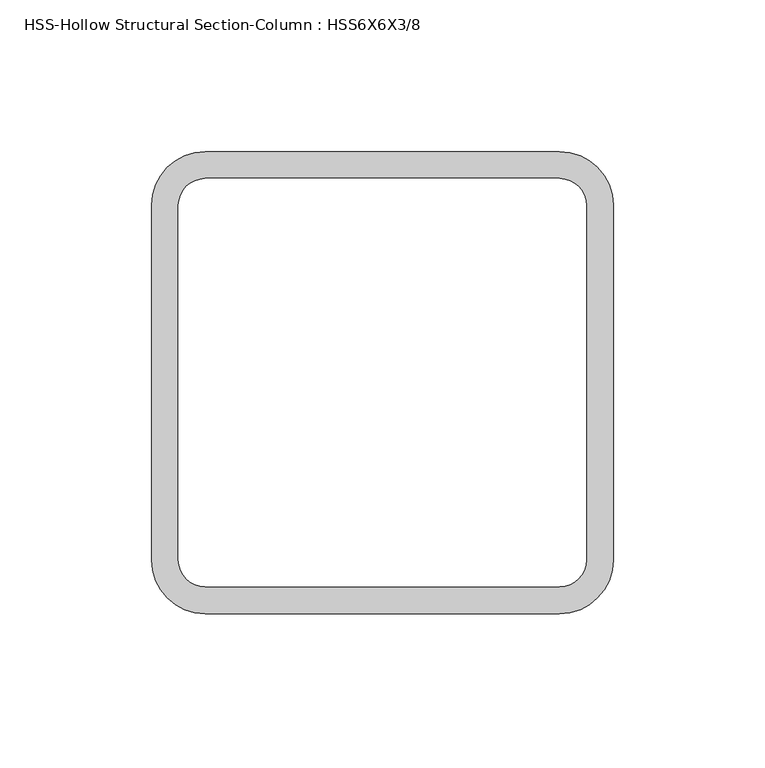
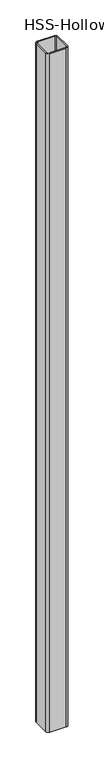
"""IFC4 building model written with IfcOpenShell, lengths in millimetres: column geometry, HSS-Hollow Structural Section-Column : HSS6X6X3/8."""

from ifc_helpers import new_model, si_unit, point, frame, frame_2d, origin, place, context, project, spatial, polyline, circle_curve, trimmed, segment, composite_curve, outline, extrude, source, transform, mapped, element, save


def hss_hollow_structural_section_column_hss6x6x3_8_7760a8ad(model_context):
    return source(origin(), model_context, "Body", "SweptSolid", [
        extrude(outline(composite_curve([segment(trimmed(circle_curve(frame_2d((58.4708, 58.4708)), 17.7292), [point((58.4708, 76.2))], [point((76.2, 58.4708))], False, "CARTESIAN"), True, "CONTINUOUS"), segment(polyline([(76.2, 58.4708), (76.2, -58.4708)]), True, "CONTINUOUS"), segment(trimmed(circle_curve(frame_2d((58.4708, -58.4708)), 17.7292), [point((76.2, -58.4708))], [point((58.4708, -76.2))], False, "CARTESIAN"), True, "CONTINUOUS"), segment(polyline([(58.4708, -76.2), (-58.4708, -76.2)]), True, "CONTINUOUS"), segment(trimmed(circle_curve(frame_2d((-58.4708, -58.4708)), 17.7292), [point((-58.4708, -76.2))], [point((-76.2, -58.4708))], False, "CARTESIAN"), True, "CONTINUOUS"), segment(polyline([(-76.2, -58.4708), (-76.2, 58.4708)]), True, "CONTINUOUS"), segment(trimmed(circle_curve(frame_2d((-58.4708, 58.4708)), 17.7292), [point((-76.2, 58.4708))], [point((-58.4708, 76.2))], False, "CARTESIAN"), True, "CONTINUOUS"), segment(polyline([(-58.4708, 76.2), (58.4708, 76.2)]), True, "CONTINUOUS")], self_intersect=False), holes=[composite_curve([segment(polyline([(58.4708, 67.3354), (-58.4708, 67.3354)]), True, "CONTINUOUS"), segment(trimmed(circle_curve(frame_2d((-58.4708, 58.4708)), 8.8646), [point((-58.4708, 67.3354))], [point((-67.3354, 58.4708))], True, "CARTESIAN"), True, "CONTINUOUS"), segment(polyline([(-67.3354, 58.4708), (-67.3354, -58.4708)]), True, "CONTINUOUS"), segment(trimmed(circle_curve(frame_2d((-58.4708, -58.4708)), 8.8646), [point((-67.3354, -58.4708))], [point((-58.4708, -67.3354))], True, "CARTESIAN"), True, "CONTINUOUS"), segment(polyline([(-58.4708, -67.3354), (58.4708, -67.3354)]), True, "CONTINUOUS"), segment(trimmed(circle_curve(frame_2d((58.4708, -58.4708)), 8.8646), [point((58.4708, -67.3354))], [point((67.3354, -58.4708))], True, "CARTESIAN"), True, "CONTINUOUS"), segment(polyline([(67.3354, -58.4708), (67.3354, 58.4708)]), True, "CONTINUOUS"), segment(trimmed(circle_curve(frame_2d((58.4708, 58.4708)), 8.8646), [point((67.3354, 58.4708))], [point((58.4708, 67.3354))], True, "CARTESIAN"), True, "CONTINUOUS")], self_intersect=False)]), frame((0.0, 0.0, 12566.65), z_axis=(0.0, 0.0, 1.0), x_axis=(1.0, 0.0, 0.0)), (0.0, 0.0, 1.0), 5060.95),
    ])


if __name__ == "__main__":
    model = new_model("IFC4")
    model_context = context("Model", 3, world=origin())
    ifc_project = project(units=[si_unit("LENGTHUNIT", "METRE", prefix="MILLI")], contexts=[model_context])
    site = spatial("IfcSite", under=ifc_project)
    building = spatial("IfcBuilding", under=site)
    placement = place(None, origin())
    hss_hollow_structural_section_column_hss6x6x3_8_shape = hss_hollow_structural_section_column_hss6x6x3_8_7760a8ad(model_context)
    element("IfcColumn", 1, ObjectType="HSS-Hollow Structural Section-Column : HSS6X6X3/8", at=placement, inside=building, context=model_context, shape_type="MappedRepresentation", body=[
        mapped(hss_hollow_structural_section_column_hss6x6x3_8_shape, transform((0.0, 0.0, 0.0), x_axis=(1.0, 0.0, 0.0), y_axis=(0.0, 1.0, 0.0), z_axis=(0.0, 0.0, 1.0))),
    ])
    save(model, "model.ifc")

# Revit data of these elements
# Type "HSS-Hollow Structural Section-Column : HSS6X6X3/8"
#   Assembly Code = "B10"
#   Shape = "Square"
#   W = 27.4
#   Ht = 0' - 6"
#   b = 0' - 6"
#   kr = 0' - 0.698"
#   t = 0' - 0.349"
#   A = 0.0526389 SF
#   Structural Material [instance default] = Steel ASTM A500, Grade B, Rectangular and Square
# Element 1 (IfcColumn, "HSS-Hollow Structural Section-Column : HSS6X6X3/8")
#   Materials on its faces: "Steel ASTM A500, Grade B, Rectangular and Square"
# Materials
#   "Steel ASTM A500, Grade B, Rectangular and Square": class "Metal", colour RGB 199 199 199, transparency 0, Description = "Carbon steel", Cost = 0
